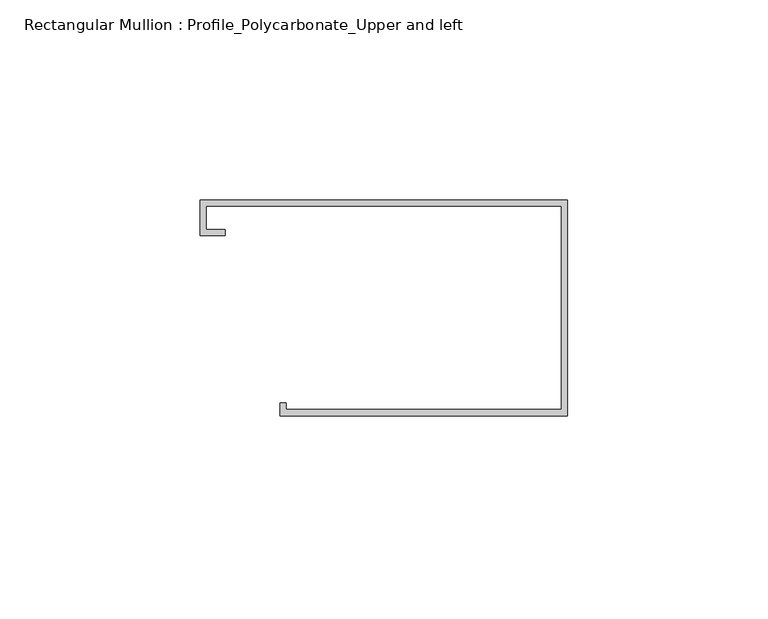
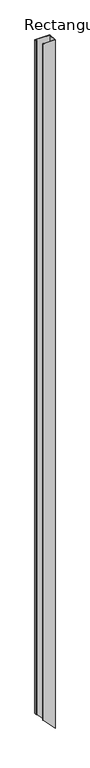
"""IFC4 building model written with IfcOpenShell, lengths in millimetres: member geometry, Rectangular Mullion : Profile_Polycarbonate_Upper and left."""

from ifc_helpers import new_model, si_unit, origin, place, context, project, spatial, faceted_brep, source, transform, mapped, element, save


def rectangular_mullion_profile_polycarbonate_upper_and_left_365aef25(model_context):
    return source(origin(), model_context, "Body", "Brep", [
        faceted_brep([(0.0, 28.984575, 0.0), (-91.9988, 28.984575, 0.0), (-91.9988, 19.992975, 0.0), (-85.6488, 19.992975, 0.0), (-85.6488, 21.580475, 0.0), (-90.4113, 21.580475, 0.0), (-90.4113, 27.397075, 0.0), (-1.5875, 27.397075, 0.0), (-1.5875, -23.428325, 0.0), (-70.3961, -23.428325, 0.0), (-70.3961, -21.840825, 0.0), (-71.9836, -21.840825, 0.0), (-71.9836, -25.015825, 0.0), (0.0, -25.015825, 0.0), (0.0, 28.984575, -4446.190625), (-91.9988, 28.984575, -4350.2787162), (-91.9988, 19.992975, -4350.2787162), (-85.6488, 19.992975, -4356.8988093), (-85.6488, 21.580475, -4356.8988093), (-90.4113, 21.580475, -4351.9337395), (-90.4113, 27.397075, -4351.9337395), (-1.5875, 27.397075, -4444.5356017), (-1.5875, -23.428325, -4444.5356017), (-70.3961, -23.428325, -4372.8002729), (-70.3961, -21.840825, -4372.8002729), (-71.9836, -21.840825, -4371.1452497), (-71.9836, -25.015825, -4371.1452497), (0.0, -25.015825, -4446.190625)], [[[0, 1, 2, 3, 4, 5, 6, 7, 8, 9, 10, 11, 12, 13]], [[1, 0, 14, 15]], [[2, 1, 15, 16]], [[3, 2, 16, 17]], [[4, 3, 17, 18]], [[5, 4, 18, 19]], [[6, 5, 19, 20]], [[7, 6, 20, 21]], [[8, 7, 21, 22]], [[9, 8, 22, 23]], [[10, 9, 23, 24]], [[11, 10, 24, 25]], [[12, 11, 25, 26]], [[13, 12, 26, 27]], [[0, 13, 27, 14]], [[14, 27, 26, 25, 24, 23, 22, 21, 20, 19, 18, 17, 16, 15]]]),
    ])


if __name__ == "__main__":
    model = new_model("IFC4")
    model_context = context("Model", 3, world=origin())
    ifc_project = project(units=[si_unit("LENGTHUNIT", "METRE", prefix="MILLI")], contexts=[model_context])
    site = spatial("IfcSite", under=ifc_project)
    building = spatial("IfcBuilding", under=site)
    placement = place(None, origin())
    rectangular_mullion_profile_polycarbonate_upper_and_left_shape = rectangular_mullion_profile_polycarbonate_upper_and_left_365aef25(model_context)
    element("IfcMember", 1, ObjectType="Rectangular Mullion : Profile_Polycarbonate_Upper and left", at=placement, inside=building, context=model_context, shape_type="MappedRepresentation", body=[
        mapped(rectangular_mullion_profile_polycarbonate_upper_and_left_shape, transform((0.0, 0.0, 0.0), x_axis=(1.0, 0.0, 0.0), y_axis=(0.0, 1.0, 0.0), z_axis=(0.0, 0.0, 1.0))),
    ])
    save(model, "model.ifc")

# Revit data of these elements
# Type "Rectangular Mullion : Profile_Polycarbonate_Upper and left"
#   built-in parameter 1007322 = 0.177167 (stored number, unit not read)
#   built-in parameter 1007321 = 0.00520833 (stored number, unit not read)
#   built-in parameter 1007320 = 0 (stored number, unit not read)
